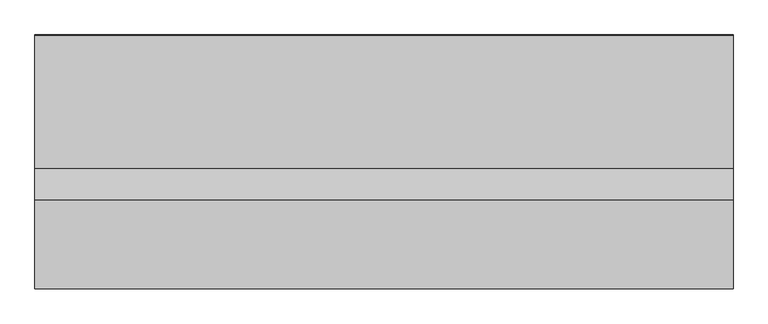
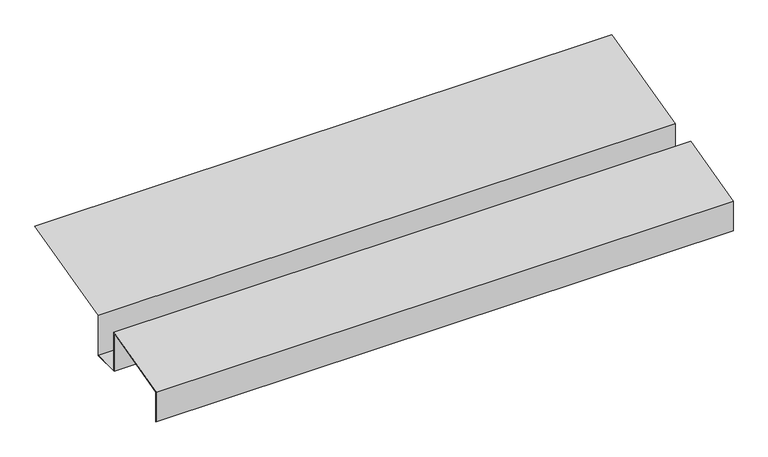
"""IFC4 building model written with IfcOpenShell, lengths in millimetres: proxy geometry, Gutter Adherance Membrane 34392 : Gutter Adherance Membrane 34392."""

from ifc_helpers import new_model, si_unit, frame, origin, place, context, project, spatial, polyline, outline, extrude, source, transform, mapped, element, save


def generic_models_997b00de(model_context):
    return source(origin(), model_context, "Body", "SweptSolid", [
        extrude(outline(polyline([(-5594.6354292, 42634.3617562), (-5594.6354292, 42743.8113639), (-5340.7070312, 42809.4422799), (-5340.7070312, 42668.34375), (-5248.1181651, 42668.34375), (-5248.1181651, 42816.2751118), (-4867.1925603, 42911.3566499), (-4866.8081055, 42909.8164062), (-5246.5306641, 42815.0351562), (-5246.5306641, 42666.75625), (-5342.2945313, 42666.75625), (-5342.2945313, 42807.3923035), (-5593.0479293, 42742.5820053), (-5593.0479293, 42634.3617562), (-5594.6354292, 42634.3617562)])), frame((12382.7678845, 0.0, 0.0), z_axis=(1.0, 0.0, 0.0), x_axis=(0.0, 1.0, 0.0)), (0.0, 0.0, 1.0), 2000.25),
    ])


if __name__ == "__main__":
    model = new_model("IFC4")
    model_context = context("Model", 3, world=origin())
    ifc_project = project(units=[si_unit("LENGTHUNIT", "METRE", prefix="MILLI")], contexts=[model_context])
    site = spatial("IfcSite", under=ifc_project)
    building = spatial("IfcBuilding", under=site)
    placement = place(None, origin())
    generic_models_shape = generic_models_997b00de(model_context)
    element("IfcBuildingElementProxy", 1, Name="Gutter Adherance Membrane 34392 : Gutter Adherance Membrane 34392", ObjectType="Gutter Adherance Membrane 34392 : Gutter Adherance Membrane 34392", at=placement, inside=building, context=model_context, shape_type="MappedRepresentation", body=[
        mapped(generic_models_shape, transform((0.0, 0.0, 0.0), x_axis=(1.0, 0.0, 0.0), y_axis=(0.0, 1.0, 0.0), z_axis=(0.0, 0.0, 1.0))),
    ])
    save(model, "model.ifc")

# Revit data of these elements
# Type "Gutter Adherance Membrane 34392 : Gutter Adherance Membrane 34392"
#   NameOverride = "Gutter Adherance Membrane"
# Element 1 (IfcBuildingElementProxy, "Gutter Adherance Membrane 34392 : Gutter Adherance Membrane 34392")
#   Materials on its faces: "SELF ADHERED MEMBRANE W/ END DAMS WHERE POSSIBLE"
# Materials
#   "SELF ADHERED MEMBRANE W/ END DAMS WHERE POSSIBLE": class "Unassigned", colour RGB 255 255 127, transparency 0
